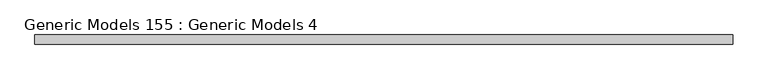
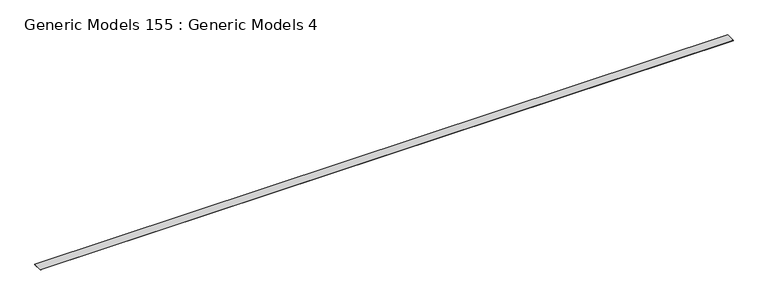
"""IFC4 building model written with IfcOpenShell, lengths in millimetres: proxy geometry, Generic Models 155 : Generic Models 4."""

from ifc_helpers import new_model, si_unit, frame, origin, place, context, project, spatial, polyline, outline, extrude, source, transform, mapped, element, save


def generic_models_155_generic_models_4_37d96fb3(model_context):
    return source(origin(), model_context, "Body", "SweptSolid", [
        extrude(outline(polyline([(-287.5914237, 6877.7114142), (-287.5914237, 6980.8708981), (7599.1085763, 6980.8708981), (7599.1085763, 6877.7114142), (-287.5914237, 6877.7114142)])), frame((0.0, 0.0, 124211.4007841), z_axis=(0.0, 0.0, 1.0), x_axis=(1.0, 0.0, 0.0)), (0.0, 0.0, 1.0), 1.3753749),
        extrude(outline(polyline([(-287.5914237, 6877.7114142), (-287.5914237, 6980.8708981), (7599.1085763, 6980.8708981), (7599.1085763, 6877.7114142), (-287.5914237, 6877.7114142)])), frame((0.0, 0.0, 124208.0071259), z_axis=(0.0, 0.0, 1.0), x_axis=(1.0, 0.0, 0.0)), (0.0, 0.0, 1.0), 1.3753749),
    ])


if __name__ == "__main__":
    model = new_model("IFC4")
    model_context = context("Model", 3, world=origin())
    ifc_project = project(units=[si_unit("LENGTHUNIT", "METRE", prefix="MILLI")], contexts=[model_context])
    site = spatial("IfcSite", under=ifc_project)
    building = spatial("IfcBuilding", under=site)
    placement = place(None, origin())
    generic_models_155_generic_models_4_shape = generic_models_155_generic_models_4_37d96fb3(model_context)
    element("IfcBuildingElementProxy", 1, Name="Generic Models 155 : Generic Models 4", ObjectType="Generic Models 155 : Generic Models 4", at=placement, inside=building, context=model_context, shape_type="MappedRepresentation", body=[
        mapped(generic_models_155_generic_models_4_shape, transform((0.0, 0.0, 0.0), x_axis=(1.0, 0.0, 0.0), y_axis=(0.0, 1.0, 0.0), z_axis=(0.0, 0.0, 1.0))),
    ])
    save(model, "model.ifc")

# Revit data of these elements
# Element 1 (IfcBuildingElementProxy, "Generic Models 155 : Generic Models 4")
#   Materials on its faces: "_BED OF SEALANT (ABOVE/BELOW FLASHING)"
# Materials
#   "_BED OF SEALANT (ABOVE/BELOW FLASHING)": class "Generic", colour RGB 253 192 103, transparency 0, Cost = 0
